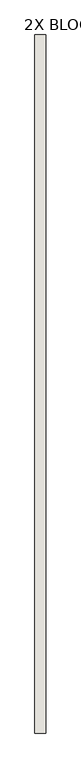
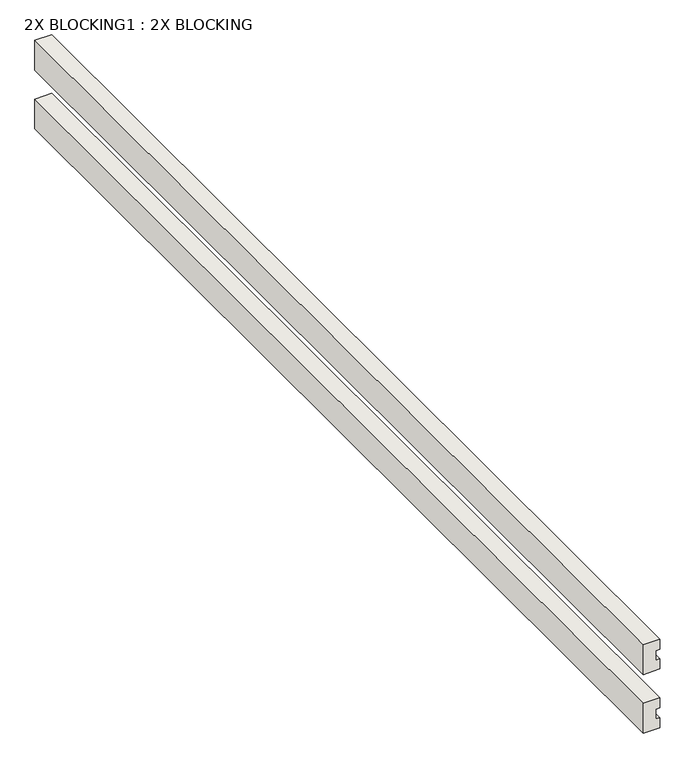
"""IFC4 building model written with IfcOpenShell, lengths in millimetres: wall geometry, 2X BLOCKING1 : 2X BLOCKING."""

from ifc_helpers import new_model, si_unit, frame, origin, place, context, project, spatial, polyline, outline, extrude, source, transform, mapped, element, save


def wall_2x_blocking1_2x_blocking_4b3cc987(model_context):
    return source(origin(), model_context, "Body", "SweptSolid", [
        extrude(outline(polyline([(2556.4977839, 19663.5620052), (2590.8, 19663.5620052), (2590.8, 19609.5870052), (2489.2, 19609.5870052), (2489.2, 19663.5620052), (2523.5022161, 19663.5620052), (2523.5022161, 19650.8620052), (2556.4977839, 19650.8620052), (2556.4977839, 19663.5620052)])), frame((0.0, -3415.0384634, 0.0), z_axis=(0.0, 1.0, 0.0), x_axis=(0.0, 0.0, 1.0)), (0.0, 0.0, 1.0), 3403.6),
        extrude(outline(polyline([(2756.5227839, 19663.5620052), (2790.825, 19663.5620052), (2790.825, 19609.5870052), (2689.225, 19609.5870052), (2689.225, 19663.5620052), (2723.5272161, 19663.5620052), (2723.5272161, 19650.8620052), (2756.5227839, 19650.8620052), (2756.5227839, 19663.5620052)])), frame((0.0, -3415.0384634, 0.0), z_axis=(0.0, 1.0, 0.0), x_axis=(0.0, 0.0, 1.0)), (0.0, 0.0, 1.0), 3403.6),
    ])


if __name__ == "__main__":
    model = new_model("IFC4")
    model_context = context("Model", 3, world=origin())
    ifc_project = project(units=[si_unit("LENGTHUNIT", "METRE", prefix="MILLI")], contexts=[model_context])
    site = spatial("IfcSite", under=ifc_project)
    building = spatial("IfcBuilding", under=site)
    placement = place(None, origin())
    wall_2x_blocking1_2x_blocking_shape = wall_2x_blocking1_2x_blocking_4b3cc987(model_context)
    element("IfcWall", 1, ObjectType="2X BLOCKING1 : 2X BLOCKING", at=placement, inside=building, context=model_context, shape_type="MappedRepresentation", body=[
        mapped(wall_2x_blocking1_2x_blocking_shape, transform((0.0, 0.0, 0.0), x_axis=(1.0, 0.0, 0.0), y_axis=(0.0, 1.0, 0.0), z_axis=(0.0, 0.0, 1.0))),
    ])
    save(model, "model.ifc")

# Revit data of these elements
# Type "2X BLOCKING1 : 2X BLOCKING"
#   Structural Material = 2 X BLOCKING
# Element 1 (IfcWall, "2X BLOCKING1 : 2X BLOCKING")
#   Materials on its faces: "BLOCKING AS NEEDED"
# Materials
#   "2 X BLOCKING": class "Wood", colour RGB 234 198 147, transparency 0, Description = "Pinus Echinata", Cost = 0
#   "BLOCKING AS NEEDED": class "Wood", colour RGB 234 198 147, transparency 0, Description = "Pinus Echinata", Cost = 0
